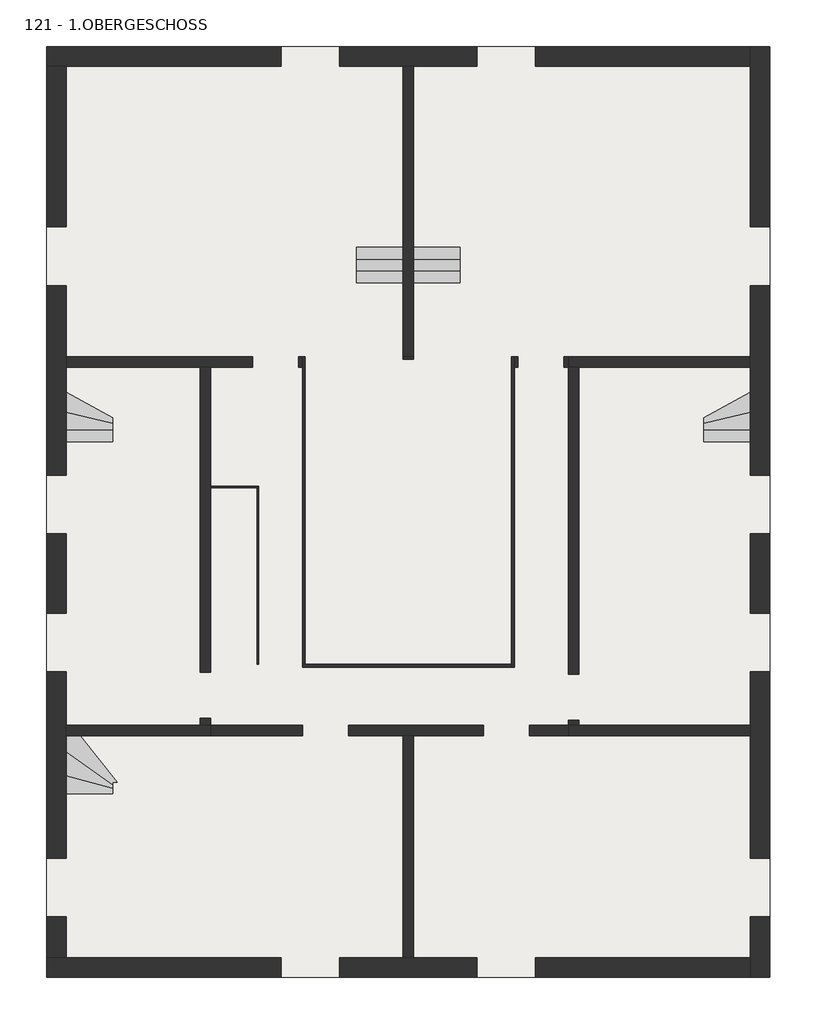
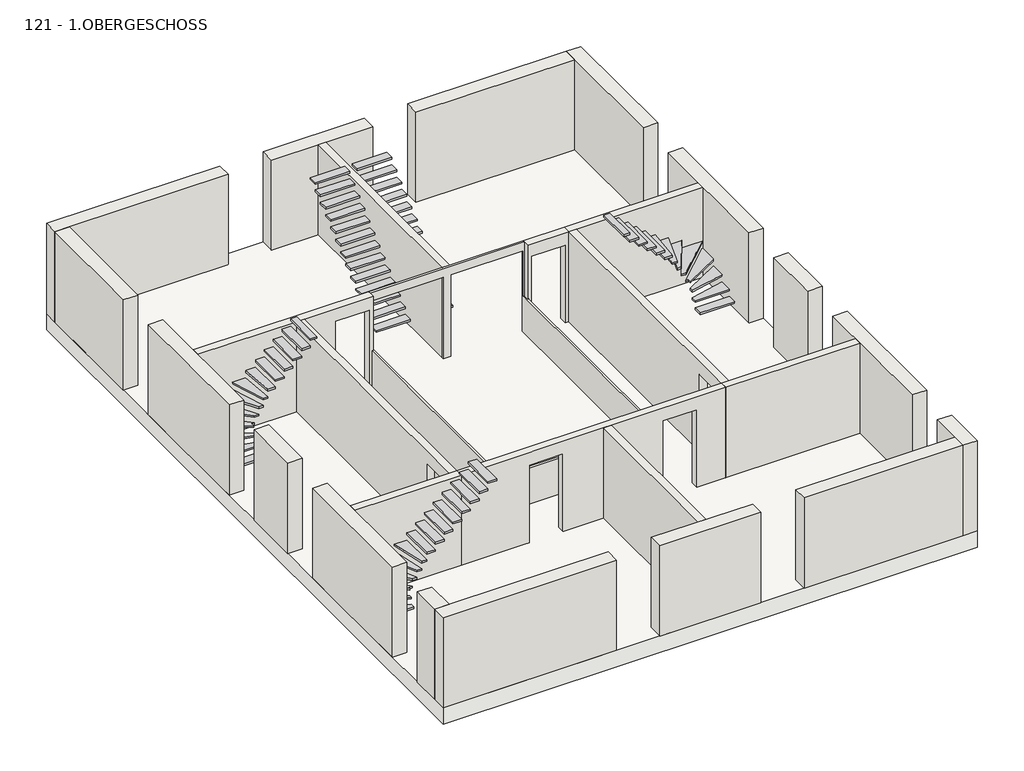
# One storey: 20 walls, 10 stairs, 1 slab.
# Revit data of these elements (continued)
# Type "  97010 :   97010" (continued)
#   HasNonSkidSurface = no
# Type "  97882 :   97882"
#   Abrechnungsart = "St"
#   Allright_Bauteil_ID = "0121Tre0785065280"
#   Codetext = "TR-MASSIV-GER\\"
#   Material = "Stahlbeton"
#   Objektname = "Treppe"
#   NameOverride = " "
#   Reference = "STB-Treppe"
#   ThermalTransmittance = 0.0000 BTU/(h·ft²·°F)
#   NosingLength = 0.000 m
#   NumberOfRiser = 14
#   NumberOfTreads = 13
#   RiserHeight = 2.021 m
#   TreadLength = 2.300 m
#   IsExternal = no
#   FireExit = no
#   HandicapAccessible = no
#   HasNonSkidSurface = no
# Type "  98300 :   98300"
#   Abrechnungsart = "St"
#   Allright_Bauteil_ID = "0121Tre0785065278"
#   Codetext = "TR-MASSIV-GER\\"
#   Material = "Stahlbeton"
#   Objektname = "Treppe"
#   NameOverride = " "
#   Reference = "STB-Treppe"
#   ThermalTransmittance = 0.0000 BTU/(h·ft²·°F)
#   NosingLength = 0.000 m
#   NumberOfRiser = 14
#   NumberOfTreads = 13
#   RiserHeight = 2.021 m
#   TreadLength = 2.300 m
#   IsExternal = no
#   FireExit = no
#   HandicapAccessible = no
#   HasNonSkidSurface = no
# Type "  98728 :   98728"
#   Abrechnungsart = "St"
#   Allright_Bauteil_ID = "0121Tre0785070507"
#   Material = "Stahlbeton"
#   Objektname = "Treppe"
#   NameOverride = " "
#   ThermalTransmittance = 0.0000 BTU/(h·ft²·°F)
#   NosingLength = 0.000 m
#   NumberOfRiser = 14
#   NumberOfTreads = 13
#   RiserHeight = 2.021 m
#   TreadLength = 2.300 m
#   IsExternal = no
#   FireExit = no
#   HandicapAccessible = no
#   HasNonSkidSurface = no
# Type "  99154 :   99154"
#   Abrechnungsart = "St"
#   Allright_Bauteil_ID = "0121Tre0785070829"
#   Material = "Stahlbeton"
#   Objektname = "Treppe"
#   NameOverride = " "
#   ThermalTransmittance = 0.0000 BTU/(h·ft²·°F)
#   NosingLength = 0.000 m
#   NumberOfRiser = 14
#   NumberOfTreads = 13
#   RiserHeight = 2.021 m
#   TreadLength = 2.300 m
#   IsExternal = no
#   FireExit = no
#   HandicapAccessible = no
#   HasNonSkidSurface = no
# Type "  149542 :   149542"
#   Abrechnungsart = "St"
#   Allright_Bauteil_ID = "0131Tre0659044515"
#   Material = "Stahlbeton"
#   Objektname = "Treppe"
#   NameOverride = " "
#   ThermalTransmittance = 0.0000 BTU/(h·ft²·°F)
#   NosingLength = 0.000 m
#   NumberOfRiser = 14
#   NumberOfTreads = 14
#   RiserHeight = 2.000 m
#   TreadLength = 2.300 m
#   IsExternal = no
#   FireExit = no
#   HandicapAccessible = no
#   HasNonSkidSurface = no
# Type "  150414 :   150414"
#   Abrechnungsart = "St"
#   Allright_Bauteil_ID = "0131Tre0659044575"
#   Codetext = "TR-MASSIV-GER\\"
#   Material = "Stahlbeton"
#   Objektname = "Treppe"
#   NameOverride = " "
#   Reference = "STB-Treppe"
#   ThermalTransmittance = 0.0000 BTU/(h·ft²·°F)
#   NosingLength = 0.000 m
#   NumberOfRiser = 14
#   NumberOfTreads = 13
#   RiserHeight = 2.021 m
#   TreadLength = 2.300 m
#   IsExternal = no
#   FireExit = no
#   HandicapAccessible = no
#   HasNonSkidSurface = no
# Type "  150832 :   150832"
#   Abrechnungsart = "St"
#   Allright_Bauteil_ID = "0131Tre0659044593"
#   Codetext = "TR-MASSIV-GER\\"
#   Material = "Stahlbeton"
#   Objektname = "Treppe"
#   NameOverride = " "
#   Reference = "STB-Treppe"
#   ThermalTransmittance = 0.0000 BTU/(h·ft²·°F)
#   NosingLength = 0.000 m
#   NumberOfRiser = 14
#   NumberOfTreads = 13
#   RiserHeight = 2.021 m
#   TreadLength = 2.300 m
#   IsExternal = no
#   FireExit = no
#   HandicapAccessible = no
#   HasNonSkidSurface = no
# Type "  151260 :   151260"
#   Abrechnungsart = "St"
#   Allright_Bauteil_ID = "0131Tre0659044533"
#   Material = "Stahlbeton"
#   Objektname = "Treppe"
#   NameOverride = " "
#   ThermalTransmittance = 0.0000 BTU/(h·ft²·°F)
#   NosingLength = 0.000 m
#   NumberOfRiser = 14
#   NumberOfTreads = 13
#   RiserHeight = 2.021 m
#   TreadLength = 2.300 m
#   IsExternal = no
#   FireExit = no
#   HandicapAccessible = no
#   HasNonSkidSurface = no
# Type "  151686 :   151686"
#   Abrechnungsart = "St"
#   Allright_Bauteil_ID = "0131Tre0659044570"
#   Material = "Stahlbeton"
#   Objektname = "Treppe"
#   NameOverride = " "
#   ThermalTransmittance = 0.0000 BTU/(h·ft²·°F)
#   NosingLength = 0.000 m
#   NumberOfRiser = 14
#   NumberOfTreads = 13
#   RiserHeight = 2.021 m
#   TreadLength = 2.300 m
#   IsExternal = no
#   FireExit = no
#   HandicapAccessible = no
#   HasNonSkidSurface = no
# Type " :1152"
#   Layers, outside or top first: 0.380 m "holzschalung" (function 1)
# Type " :1161"
#   Layers, outside or top first: 0.380 m "holzschalung" (function 1)
# Type " :1164"
#   Layers, outside or top first: 0.380 m "holzschalung" (function 1)
# Type " :1165"
#   Layers, outside or top first: 0.380 m "holzschalung" (function 1)
# Type " :1166"
#   Layers, outside or top first: 0.050 m "glas" (function 1)
# Type "Holzwand:1150"
#   ThermalTransmittance = 0.0000 BTU/(h·ft²·°F)
#   Combustible = no
#   Compartmentation = no
#   Layers, outside or top first: 0.200 m "holzschalung" (function 1)
# Type "Holzwand:1151"
#   ThermalTransmittance = 0.0000 BTU/(h·ft²·°F)
#   Combustible = no
#   Compartmentation = no
#   Layers, outside or top first: 0.200 m "holzschalung" (function 1)
# Type "Holzwand:1153"
#   ThermalTransmittance = 0.0000 BTU/(h·ft²·°F)
#   Combustible = no
#   Compartmentation = no
#   Layers, outside or top first: 0.200 m "holzschalung" (function 1)
# Type "Holzwand:1154"
#   ThermalTransmittance = 0.0000 BTU/(h·ft²·°F)
#   Combustible = no
#   Compartmentation = no
#   Layers, outside or top first: 0.030 m "holzschalung" (function 1)
# Type "Holzwand:1155"
#   ThermalTransmittance = 0.0000 BTU/(h·ft²·°F)
#   Combustible = no
#   Compartmentation = no
#   Layers, outside or top first: 0.030 m "holzschalung" (function 1)
# Type "Holzwand:1156"
#   ThermalTransmittance = 0.0000 BTU/(h·ft²·°F)
#   Combustible = no
#   Compartmentation = no
#   Layers, outside or top first: 0.200 m "holzschalung" (function 1)
# Type "Holzwand:1157"
#   ThermalTransmittance = 0.0000 BTU/(h·ft²·°F)
#   Combustible = no
#   Compartmentation = no
#   Layers, outside or top first: 0.200 m "holzschalung" (function 1)
# Type "Holzwand:1158"
#   ThermalTransmittance = 0.0000 BTU/(h·ft²·°F)
#   Combustible = no
#   Compartmentation = no
#   Layers, outside or top first: 0.200 m "holzschalung" (function 1)
# Type "Holzwand:1159"
#   ThermalTransmittance = 0.0000 BTU/(h·ft²·°F)
#   Combustible = no
#   Compartmentation = no
#   Layers, outside or top first: 0.200 m "holzschalung" (function 1)
# Type "Holzwand:1160"
#   ThermalTransmittance = 0.0000 BTU/(h·ft²·°F)
#   Combustible = no
#   Compartmentation = no
#   Layers, outside or top first: 0.200 m "holzschalung" (function 1)
# Type "Holzwand:1162"
#   ThermalTransmittance = 0.0000 BTU/(h·ft²·°F)
#   Combustible = no
#   Compartmentation = no
#   Layers, outside or top first: 0.200 m "holzschalung" (function 1)
# Type "Holzwand:1163"
#   ThermalTransmittance = 0.0000 BTU/(h·ft²·°F)
#   Combustible = no
#   Compartmentation = no
#   Layers, outside or top first: 0.200 m "holzschalung" (function 1)
# Type " :1167"
#   Layers, outside or top first: 0.050 m "holzschalung" (function 1)
# Type " :1168"
#   Layers, outside or top first: 0.050 m "holzschalung" (function 1)
# Type " :1169"
#   Layers, outside or top first: 0.050 m "holzschalung" (function 1)
# Element 1 (IfcSlab, "Holzdecke 176 : Holzdecke 176")
#   IFC Predefined Type = "FLOOR"
#   Export to IFC As = "ifcslab"
#   IfcGUID = "1_9Us2eVX4OuIZjhNyqdxW"
#   Phase Created = New Construction
#   Materials on its faces: "holzschalung"
# Element 2 (IfcStair, "  97010 :   97010")
#   IFC Predefined Type = "NOTDEFINED"
#   Export to IFC As = "ifcstair"
#   IfcGUID = "2ccaodaeb6QgHPV1d4NBnA"
#   Phase Created = New Construction
#   Materials on its faces: "weiss"
# Element 3 (IfcStair, "  97882 :   97882")
#   IFC Predefined Type = "STRAIGHT_RUN_STAIR"
#   Export to IFC As = "ifcstair"
#   IfcGUID = "1nghyUHoH9yBc_lxkBTUjw"
#   Phase Created = New Construction
#   Materials on its faces: "weiss"
# Element 4 (IfcStair, "  98300 :   98300")
#   IFC Predefined Type = "STRAIGHT_RUN_STAIR"
#   Export to IFC As = "ifcstair"
#   IfcGUID = "2AC_Gmfhz1LvYwUyPOxWan"
#   Phase Created = New Construction
#   Materials on its faces: "weiss"
# Element 5 (IfcStair, "  98728 :   98728")
#   IFC Predefined Type = "NOTDEFINED"
#   Export to IFC As = "ifcstair"
#   IfcGUID = "04Edcgbk9CPwWYiYhycXFf"
#   Phase Created = New Construction
#   Materials on its faces: "weiss"
# Element 6 (IfcStair, "  99154 :   99154")
#   IFC Predefined Type = "NOTDEFINED"
#   Export to IFC As = "ifcstair"
#   IfcGUID = "1azVXxNdn2POY9VYN93ccY"
#   Phase Created = New Construction
#   Materials on its faces: "weiss"
# Element 7 (IfcStair, "  149542 :   149542")
#   IFC Predefined Type = "NOTDEFINED"
#   Export to IFC As = "ifcstair"
#   IfcGUID = "1sH4rJKnLAFOtHPnXrLkif"
#   Phase Created = New Construction
#   Materials on its faces: "weiss"
# Element 8 (IfcStair, "  150414 :   150414")
#   IFC Predefined Type = "STRAIGHT_RUN_STAIR"
#   Export to IFC As = "ifcstair"
#   IfcGUID = "3fdccs_Mj1YAyFFpBc3gyk"
#   Phase Created = New Construction
#   Materials on its faces: "weiss"
# Element 9 (IfcStair, "  150832 :   150832")
#   IFC Predefined Type = "STRAIGHT_RUN_STAIR"
#   Export to IFC As = "ifcstair"
#   IfcGUID = "2szmEZdbD3KBDvfX1Sa6Vh"
#   Phase Created = New Construction
#   Materials on its faces: "weiss"
# Element 10 (IfcStair, "  151260 :   151260")
#   IFC Predefined Type = "NOTDEFINED"
#   Export to IFC As = "ifcstair"
#   IfcGUID = "1YKyaFTbr8YR41yGjubBsl"
#   Phase Created = New Construction
#   Materials on its faces: "weiss"
# Element 11 (IfcStair, "  151686 :   151686")
#   IFC Predefined Type = "NOTDEFINED"
#   Export to IFC As = "ifcstair"
#   IfcGUID = "2KPGRYHzzCygzBebAeLtPz"
#   Phase Created = New Construction
#   Materials on its faces: "weiss"
# Element 12 (IfcWall, " :1152")
#   Export to IFC As = "ifcwall"
#   IfcGUID = "2CeDj8YZTCPx$yj4WDVOez"
#   NameOverride = " "
#   Abrechnungsart = "m³"
#   Allright_Bauteil_ID = "0121HWa0785064286"
#   Layer #1:Object Layer Attributes #1:Abrechnungsart = "m²"
#   Layer #1:Object Layer Attributes #1:Allright_Bauteil_ID = "0121Wa 0785064367"
#   Layer #1:Object Layer Attributes #1:Gewerk = "Zimmer- und Holzbauarbeiten"
#   Layer #1:Object Layer Attributes #1:Material = "k.Ausw."
#   Layer #1:Object Layer Attributes #1:Objektname = "Wand"
#   Layer #1:Object Layer Attributes #1:Status = "Neubau"
#   MEP Wandtyp = "HO-WA-HSW\\"
#   Objektname = "Gesamtwand"
#   built-in parameter 1001111 = 0.505 m
#   Top Offset = 0.000 m
#   Base Offset = 0.505 m
#   Unconnected Height = 2.500 m
#   wall height = 2.500 m
#   Layer #1:Object Layer Attributes #1:2D Interaktion = yes
#   Phase Created = New Construction
#   Base Constraint = 121 - 1.OBERGESCHOSS
#   Materials on its faces: "holzschalung"
# Element 13 (IfcWall, " :1161")
#   Export to IFC As = "ifcwall"
#   IfcGUID = "2TnImcbz91shb3jN7Wgb8B"
#   Comments = "OG Sued"
#   Mark = "OG Sued"
#   NameOverride = " "
#   Abrechnungsart = "m³"
#   Allright_Bauteil_ID = "0121HWa0785064349"
#   Layer #1:Object Layer Attributes #1:Abrechnungsart = "m²"
#   Layer #1:Object Layer Attributes #1:Allright_Bauteil_ID = "0121Wa 0785064397"
#   Layer #1:Object Layer Attributes #1:Gewerk = "Zimmer- und Holzbauarbeiten"
#   Layer #1:Object Layer Attributes #1:Material = "k.Ausw."
#   Layer #1:Object Layer Attributes #1:Objektname = "Wand"
#   Layer #1:Object Layer Attributes #1:Status = "Neubau"
#   MEP Wandtyp = "HO-WA-HSW\\"
#   Objektname = "Gesamtwand"
#   built-in parameter 1001111 = 0.505 m
#   Top Offset = 0.000 m
#   Base Offset = 0.505 m
#   Unconnected Height = 2.500 m
#   wall height = 2.500 m
#   Layer #1:Object Layer Attributes #1:2D Interaktion = yes
#   Phase Created = New Construction
#   Base Constraint = 121 - 1.OBERGESCHOSS
#   Materials on its faces: "holzschalung"
# Element 14 (IfcWall, " :1164")
#   Export to IFC As = "ifcwall"
#   IfcGUID = "1tWRh4hxLAdASVw4VNE3to"
#   NameOverride = " "
#   Abrechnungsart = "m³"
#   Allright_Bauteil_ID = "0121HWa0785092952"
#   Layer #1:Object Layer Attributes #1:Abrechnungsart = "m²"
#   Layer #1:Object Layer Attributes #1:Allright_Bauteil_ID = "0121Wa 0785092986"
#   Layer #1:Object Layer Attributes #1:Gewerk = "Zimmer- und Holzbauarbeiten"
#   Layer #1:Object Layer Attributes #1:Material = "k.Ausw."
#   Layer #1:Object Layer Attributes #1:Objektname = "Wand"
#   Layer #1:Object Layer Attributes #1:Status = "Neubau"
#   MEP Wandtyp = "HO-WA-HSW\\"
#   Objektname = "Gesamtwand"
#   built-in parameter 1001111 = 0.505 m
#   Top Offset = 0.000 m
#   Base Offset = 0.505 m
#   Unconnected Height = 2.500 m
#   wall height = 2.500 m
#   Layer #1:Object Layer Attributes #1:2D Interaktion = yes
#   Phase Created = New Construction
#   Base Constraint = 121 - 1.OBERGESCHOSS
#   Materials on its faces: "holzschalung"
# Element 15 (IfcWall, " :1165")
#   Export to IFC As = "ifcwall"
#   IfcGUID = "1HE73MTmDEEBf4AV7ughZ8"
#   NameOverride = " "
#   Abrechnungsart = "m³"
#   Allright_Bauteil_ID = "0121HWa0785097898"
#   Layer #1:Object Layer Attributes #1:Abrechnungsart = "m²"
#   Layer #1:Object Layer Attributes #1:Allright_Bauteil_ID = "0121Wa 0785097934"
#   Layer #1:Object Layer Attributes #1:Gewerk = "Zimmer- und Holzbauarbeiten"
#   Layer #1:Object Layer Attributes #1:Material = "k.Ausw."
#   Layer #1:Object Layer Attributes #1:Objektname = "Wand"
#   Layer #1:Object Layer Attributes #1:Status = "Neubau"
#   MEP Wandtyp = "HO-WA-HSW\\"
#   Objektname = "Gesamtwand"
#   built-in parameter 1001111 = 0.505 m
#   Top Offset = 0.000 m
#   Base Offset = 0.505 m
#   Unconnected Height = 2.500 m
#   wall height = 2.500 m
#   Layer #1:Object Layer Attributes #1:2D Interaktion = yes
#   Phase Created = New Construction
#   Base Constraint = 121 - 1.OBERGESCHOSS
#   Materials on its faces: "holzschalung"
# Element 16 (IfcWall, " :1166")
#   Export to IFC As = "ifcwall"
#   IfcGUID = "0t2qqx1kvDZPNPdKl4bfzP"
#   NameOverride = " "
#   Abrechnungsart = "m³"
#   Allright_Bauteil_ID = "0121HWa0785064296"
#   Layer #1:Object Layer Attributes #1:Abrechnungsart = "m²"
#   Layer #1:Object Layer Attributes #1:Allright_Bauteil_ID = "0121Wa 0785064386"
#   Layer #1:Object Layer Attributes #1:Gewerk = "Zimmer- und Holzbauarbeiten"
#   Layer #1:Object Layer Attributes #1:Material = "k.Ausw."
#   Layer #1:Object Layer Attributes #1:Objektname = "Wand"
#   Layer #1:Object Layer Attributes #1:Status = "Neubau"
#   MEP Wandtyp = "HO-WA-HSW\\"
#   Objektname = "Gesamtwand"
#   built-in parameter 1001111 = 0.505 m
#   Top Offset = 0.000 m
#   Base Offset = 0.505 m
#   Unconnected Height = 2.500 m
#   wall height = 2.500 m
#   Layer #1:Object Layer Attributes #1:2D Interaktion = yes
#   Phase Created = New Construction
#   Base Constraint = 121 - 1.OBERGESCHOSS
#   Materials on its faces: "glas"
# Element 17 (IfcWall, "Holzwand:1150")
#   Export to IFC As = "ifcwall"
#   IfcGUID = "3nZ5Mon9nBjwoRgvyoor9a"
#   NameOverride = "Holzwand"
#   Abrechnungsart = "St"
#   Allright_Bauteil_ID = "0121HWa0785065367"
#   Bezeichnung = "Holzwand"
#   Layer #1:Object Layer Attributes #1:Abrechnungsart = "m²"
#   Layer #1:Object Layer Attributes #1:Allright_Bauteil_ID = "0121Wa 0785065369"
#   Layer #1:Object Layer Attributes #1:Bezeichnung = "Holzwand"
#   Layer #1:Object Layer Attributes #1:Codetext = "HO-WI-HSW\\"
#   Layer #1:Object Layer Attributes #1:Gewerk = "Zimmer- und Holzbauarbeiten"
#   Layer #1:Object Layer Attributes #1:Material = "Holz"
#   Layer #1:Object Layer Attributes #1:Objektname = "Wand"
#   Layer #1:Object Layer Attributes #1:Reference = "Holzwand"
#   Layer #1:Object Layer Attributes #1:Status = "Neubau"
#   MEP Wandtyp = "HO-WA-HSW\\"
#   Objektname = "Gesamtwand"
#   Reference = "Holzwand"
#   Status = "NEW"
#   built-in parameter 1001111 = 0.505 m
#   Top Offset = 0.000 m
#   Base Offset = 0.505 m
#   Unconnected Height = 2.500 m
#   wall height = 2.500 m
#   Layer #1:Object Layer Attributes #1:U-Wert = 0
#   Layer #1:Object Layer Attributes #1:2D Interaktion = yes
#   Layer #1:Object Layer Attributes #1:Außenbauteil = no
#   Layer #1:Object Layer Attributes #1:Brandabschnittsdefinierendes Bauteil = no
#   Layer #1:Object Layer Attributes #1:Brennbares Material = no
#   Layer #1:Object Layer Attributes #1:Raumhohe Wand = yes
#   Layer #1:Object Layer Attributes #1:Tragendes Bauteil = yes
#   ExtendToStructure = yes
#   IsExternal = no
#   LoadBearing = yes
#   Phase Created = New Construction
#   Base Constraint = 121 - 1.OBERGESCHOSS
#   Materials on its faces: "holzschalung"
# Element 18 (IfcWall, "Holzwand:1151")
#   Export to IFC As = "ifcwall"
#   IfcGUID = "3jE1E$NFj7vAP$vn70kdrt"
#   NameOverride = "Holzwand"
#   Abrechnungsart = "St"
#   Allright_Bauteil_ID = "0121HWa0785066899"
#   Bezeichnung = "Holzwand"
#   Layer #1:Object Layer Attributes #1:Abrechnungsart = "m²"
#   Layer #1:Object Layer Attributes #1:Allright_Bauteil_ID = "0121Wa 0785066901"
#   Layer #1:Object Layer Attributes #1:Bezeichnung = "Holzwand"
#   Layer #1:Object Layer Attributes #1:Codetext = "HO-WI-HSW\\"
#   Layer #1:Object Layer Attributes #1:Gewerk = "Zimmer- und Holzbauarbeiten"
#   Layer #1:Object Layer Attributes #1:Material = "Holz"
#   Layer #1:Object Layer Attributes #1:Objektname = "Wand"
#   Layer #1:Object Layer Attributes #1:Reference = "Holzwand"
#   Layer #1:Object Layer Attributes #1:Status = "Neubau"
#   MEP Wandtyp = "HO-WA-HSW\\"
#   Objektname = "Gesamtwand"
#   Reference = "Holzwand"
#   Status = "NEW"
#   built-in parameter 1001111 = 0.505 m
#   Top Offset = 0.000 m
#   Base Offset = 0.505 m
#   Unconnected Height = 2.500 m
#   wall height = 2.500 m
#   Layer #1:Object Layer Attributes #1:U-Wert = 0
#   Layer #1:Object Layer Attributes #1:2D Interaktion = yes
#   Layer #1:Object Layer Attributes #1:Außenbauteil = no
#   Layer #1:Object Layer Attributes #1:Brandabschnittsdefinierendes Bauteil = no
#   Layer #1:Object Layer Attributes #1:Brennbares Material = no
#   Layer #1:Object Layer Attributes #1:Raumhohe Wand = yes
#   Layer #1:Object Layer Attributes #1:Tragendes Bauteil = yes
#   ExtendToStructure = yes
#   IsExternal = no
#   LoadBearing = yes
#   Phase Created = New Construction
#   Base Constraint = 121 - 1.OBERGESCHOSS
#   Materials on its faces: "holzschalung"
# Element 19 (IfcWall, "Holzwand:1153")
#   Export to IFC As = "ifcwall"
#   IfcGUID = "1Zhxv5EALB9e6_$pCtUEXg"
#   NameOverride = "Holzwand"
#   Abrechnungsart = "St"
#   Allright_Bauteil_ID = "0121HWa0785065540"
#   Bezeichnung = "Holzwand"
#   Layer #1:Object Layer Attributes #1:Abrechnungsart = "m²"
#   Layer #1:Object Layer Attributes #1:Allright_Bauteil_ID = "0121Wa 0785065541"
#   Layer #1:Object Layer Attributes #1:Bezeichnung = "Holzwand"
#   Layer #1:Object Layer Attributes #1:Codetext = "HO-WI-HSW\\"
#   Layer #1:Object Layer Attributes #1:Gewerk = "Zimmer- und Holzbauarbeiten"
#   Layer #1:Object Layer Attributes #1:Material = "Holz"
#   Layer #1:Object Layer Attributes #1:Objektname = "Wand"
#   Layer #1:Object Layer Attributes #1:Reference = "Holzwand"
#   Layer #1:Object Layer Attributes #1:Status = "Neubau"
#   MEP Wandtyp = "HO-WA-HSW\\"
#   Objektname = "Gesamtwand"
#   Reference = "Holzwand"
#   Status = "NEW"
#   built-in parameter 1001111 = 0.505 m
#   Top Offset = 0.000 m
#   Base Offset = 0.505 m
#   Unconnected Height = 2.500 m
#   wall height = 2.500 m
#   Layer #1:Object Layer Attributes #1:U-Wert = 0
#   Layer #1:Object Layer Attributes #1:2D Interaktion = yes
#   Layer #1:Object Layer Attributes #1:Außenbauteil = no
#   Layer #1:Object Layer Attributes #1:Brandabschnittsdefinierendes Bauteil = no
#   Layer #1:Object Layer Attributes #1:Brennbares Material = no
#   Layer #1:Object Layer Attributes #1:Raumhohe Wand = yes
#   Layer #1:Object Layer Attributes #1:Tragendes Bauteil = yes
#   ExtendToStructure = yes
#   IsExternal = no
#   LoadBearing = yes
#   Phase Created = New Construction
#   Base Constraint = 121 - 1.OBERGESCHOSS
#   Materials on its faces: "holzschalung"
# Element 20 (IfcWall, "Holzwand:1154")
#   Export to IFC As = "ifcwall"
#   IfcGUID = "2MsVq3EJn0K8wHdQ6uoxnd"
#   NameOverride = "Holzwand"
#   Abrechnungsart = "St"
#   Allright_Bauteil_ID = "0121HWa0785067355"
#   Bezeichnung = "Holzwand"
#   Layer #1:Object Layer Attributes #1:Abrechnungsart = "m²"
#   Layer #1:Object Layer Attributes #1:Allright_Bauteil_ID = "0121Wa 0785067356"
#   Layer #1:Object Layer Attributes #1:Codetext = "HO-WI-HSW\\"
#   Layer #1:Object Layer Attributes #1:Gewerk = "Zimmer- und Holzbauarbeiten"
#   Layer #1:Object Layer Attributes #1:Material = "Holz"
#   Layer #1:Object Layer Attributes #1:Objektname = "Wand"
#   Layer #1:Object Layer Attributes #1:Reference = "Holzwand"
#   Layer #1:Object Layer Attributes #1:Status = "Neubau"
#   MEP Wandtyp = "HO-WA-HSW\\"
#   Objektname = "Gesamtwand"
#   Reference = "Holzwand"
#   Status = "NEW"
#   built-in parameter 1001111 = 0.505 m
#   Top Offset = 0.000 m
#   Base Offset = 0.505 m
#   Unconnected Height = 1.000 m
#   wall height = 1.000 m
#   Layer #1:Object Layer Attributes #1:U-Wert = 0
#   Layer #1:Object Layer Attributes #1:2D Interaktion = yes
#   Layer #1:Object Layer Attributes #1:Außenbauteil = no
#   Layer #1:Object Layer Attributes #1:Brandabschnittsdefinierendes Bauteil = no
#   Layer #1:Object Layer Attributes #1:Brennbares Material = no
#   Layer #1:Object Layer Attributes #1:Raumhohe Wand = yes
#   ExtendToStructure = yes
#   IsExternal = no
#   LoadBearing = yes
#   Phase Created = New Construction
#   Base Constraint = 121 - 1.OBERGESCHOSS
#   Materials on its faces: "holzschalung"
# Element 21 (IfcWall, "Holzwand:1155")
#   Export to IFC As = "ifcwall"
#   IfcGUID = "1F_ySrDsP9oP3MqXymSTVO"
#   NameOverride = "Holzwand"
#   Abrechnungsart = "St"
#   Allright_Bauteil_ID = "0121HWa0785067347"
#   Bezeichnung = "Holzwand"
#   Layer #1:Object Layer Attributes #1:Abrechnungsart = "m²"
#   Layer #1:Object Layer Attributes #1:Allright_Bauteil_ID = "0121Wa 0785067348"
#   Layer #1:Object Layer Attributes #1:Codetext = "HO-WI-HSW\\"
#   Layer #1:Object Layer Attributes #1:Gewerk = "Zimmer- und Holzbauarbeiten"
#   Layer #1:Object Layer Attributes #1:Material = "Holz"
#   Layer #1:Object Layer Attributes #1:Objektname = "Wand"
#   Layer #1:Object Layer Attributes #1:Reference = "Holzwand"
#   Layer #1:Object Layer Attributes #1:Status = "Neubau"
#   MEP Wandtyp = "HO-WA-HSW\\"
#   Objektname = "Gesamtwand"
#   Reference = "Holzwand"
#   Status = "NEW"
#   built-in parameter 1001111 = 0.505 m
#   Top Offset = 0.000 m
#   Base Offset = 0.505 m
#   Unconnected Height = 1.000 m
#   wall height = 1.000 m
#   Layer #1:Object Layer Attributes #1:U-Wert = 0
#   Layer #1:Object Layer Attributes #1:2D Interaktion = yes
#   Layer #1:Object Layer Attributes #1:Außenbauteil = no
#   Layer #1:Object Layer Attributes #1:Brandabschnittsdefinierendes Bauteil = no
#   Layer #1:Object Layer Attributes #1:Brennbares Material = no
#   Layer #1:Object Layer Attributes #1:Raumhohe Wand = yes
#   ExtendToStructure = yes
#   IsExternal = no
#   LoadBearing = yes
#   Phase Created = New Construction
#   Base Constraint = 121 - 1.OBERGESCHOSS
#   Materials on its faces: "holzschalung"
# Element 22 (IfcWall, "Holzwand:1156")
#   Export to IFC As = "ifcwall"
#   IfcGUID = "0gtwZwppj1pObqyI7HY41_"
#   NameOverride = "Holzwand"
#   Abrechnungsart = "St"
#   Allright_Bauteil_ID = "0121HWa0785064323"
#   Bezeichnung = "Holzwand"
#   Layer #1:Object Layer Attributes #1:Abrechnungsart = "m²"
#   Layer #1:Object Layer Attributes #1:Allright_Bauteil_ID = "0121Wa 0785064369"
#   Layer #1:Object Layer Attributes #1:Bezeichnung = "Holzwand"
#   Layer #1:Object Layer Attributes #1:Codetext = "HO-WI-HSW\\"
#   Layer #1:Object Layer Attributes #1:Gewerk = "Zimmer- und Holzbauarbeiten"
#   Layer #1:Object Layer Attributes #1:Material = "Holz"
#   Layer #1:Object Layer Attributes #1:Objektname = "Wand"
#   Layer #1:Object Layer Attributes #1:Reference = "Holzwand"
#   Layer #1:Object Layer Attributes #1:Status = "Neubau"
#   MEP Wandtyp = "HO-WA-HSW\\"
#   Objektname = "Gesamtwand"
#   Reference = "Holzwand"
#   Status = "NEW"
#   built-in parameter 1001111 = 0.505 m
#   Top Offset = 0.000 m
#   Base Offset = 0.505 m
#   Unconnected Height = 2.500 m
#   wall height = 2.500 m
#   Layer #1:Object Layer Attributes #1:U-Wert = 0
#   Layer #1:Object Layer Attributes #1:2D Interaktion = yes
#   Layer #1:Object Layer Attributes #1:Außenbauteil = no
#   Layer #1:Object Layer Attributes #1:Brandabschnittsdefinierendes Bauteil = no
#   Layer #1:Object Layer Attributes #1:Brennbares Material = no
#   Layer #1:Object Layer Attributes #1:Raumhohe Wand = yes
#   Layer #1:Object Layer Attributes #1:Tragendes Bauteil = yes
#   ExtendToStructure = yes
#   IsExternal = no
#   LoadBearing = yes
#   Phase Created = New Construction
#   Base Constraint = 121 - 1.OBERGESCHOSS
#   Materials on its faces: "holzschalung"
# Element 23 (IfcWall, "Holzwand:1157")
#   Export to IFC As = "ifcwall"
#   IfcGUID = "0tY6$O1l121AktLhYSWZjf"
#   NameOverride = "Holzwand"
#   Abrechnungsart = "St"
#   Allright_Bauteil_ID = "0121HWa0785064381"
#   Bezeichnung = "Holzwand"
#   Layer #1:Object Layer Attributes #1:Abrechnungsart = "m²"
#   Layer #1:Object Layer Attributes #1:Allright_Bauteil_ID = "0121Wa 0785064384"
#   Layer #1:Object Layer Attributes #1:Bezeichnung = "Holzwand"
#   Layer #1:Object Layer Attributes #1:Codetext = "HO-WI-HSW\\"
#   Layer #1:Object Layer Attributes #1:Gewerk = "Zimmer- und Holzbauarbeiten"
#   Layer #1:Object Layer Attributes #1:Material = "Holz"
#   Layer #1:Object Layer Attributes #1:Objektname = "Wand"
#   Layer #1:Object Layer Attributes #1:Reference = "Holzwand"
#   Layer #1:Object Layer Attributes #1:Status = "Neubau"
#   MEP Wandtyp = "HO-WA-HSW\\"
#   Objektname = "Gesamtwand"
#   Reference = "Holzwand"
#   Status = "NEW"
#   built-in parameter 1001111 = 0.505 m
#   Top Offset = 0.000 m
#   Base Offset = 0.505 m
#   Unconnected Height = 2.500 m
#   wall height = 2.500 m
#   Layer #1:Object Layer Attributes #1:U-Wert = 0
#   Layer #1:Object Layer Attributes #1:2D Interaktion = yes
#   Layer #1:Object Layer Attributes #1:Außenbauteil = no
#   Layer #1:Object Layer Attributes #1:Brandabschnittsdefinierendes Bauteil = no
#   Layer #1:Object Layer Attributes #1:Brennbares Material = no
#   Layer #1:Object Layer Attributes #1:Raumhohe Wand = yes
#   Layer #1:Object Layer Attributes #1:Tragendes Bauteil = yes
#   ExtendToStructure = yes
#   IsExternal = no
#   LoadBearing = yes
#   Phase Created = New Construction
#   Base Constraint = 121 - 1.OBERGESCHOSS
#   Materials on its faces: "holzschalung"
# Element 24 (IfcWall, "Holzwand:1158")
#   Export to IFC As = "ifcwall"
#   IfcGUID = "2Mr8L52dj4iP8MoJTiOa9p"
#   NameOverride = "Holzwand"
#   Abrechnungsart = "St"
#   Allright_Bauteil_ID = "0121HWa0785069286"
#   Bezeichnung = "Holzwand"
#   Layer #1:Object Layer Attributes #1:Abrechnungsart = "m²"
#   Layer #1:Object Layer Attributes #1:Allright_Bauteil_ID = "0121Wa 0785069294"
#   Layer #1:Object Layer Attributes #1:Bezeichnung = "Holzwand"
#   Layer #1:Object Layer Attributes #1:Codetext = "HO-WI-HSW\\"
#   Layer #1:Object Layer Attributes #1:Gewerk = "Zimmer- und Holzbauarbeiten"
#   Layer #1:Object Layer Attributes #1:Material = "Holz"
#   Layer #1:Object Layer Attributes #1:Objektname = "Wand"
#   Layer #1:Object Layer Attributes #1:Reference = "Holzwand"
#   Layer #1:Object Layer Attributes #1:Status = "Neubau"
#   MEP Wandtyp = "HO-WA-HSW\\"
#   Objektname = "Gesamtwand"
#   Reference = "Holzwand"
#   Status = "NEW"
#   built-in parameter 1001111 = 0.505 m
#   Top Offset = 0.000 m
#   Base Offset = 0.505 m
#   Unconnected Height = 2.500 m
#   wall height = 2.500 m
#   Layer #1:Object Layer Attributes #1:U-Wert = 0
#   Layer #1:Object Layer Attributes #1:2D Interaktion = yes
#   Layer #1:Object Layer Attributes #1:Außenbauteil = no
#   Layer #1:Object Layer Attributes #1:Brandabschnittsdefinierendes Bauteil = no
#   Layer #1:Object Layer Attributes #1:Brennbares Material = no
#   Layer #1:Object Layer Attributes #1:Raumhohe Wand = yes
#   Layer #1:Object Layer Attributes #1:Tragendes Bauteil = yes
#   ExtendToStructure = yes
#   IsExternal = no
#   LoadBearing = yes
#   Phase Created = New Construction
#   Base Constraint = 121 - 1.OBERGESCHOSS
#   Materials on its faces: "holzschalung"
# Element 25 (IfcWall, "Holzwand:1159")
#   Export to IFC As = "ifcwall"
#   IfcGUID = "36leNf4gL9OB_v358ffY76"
#   NameOverride = "Holzwand"
#   Abrechnungsart = "St"
#   Allright_Bauteil_ID = "0121HWa0785064324"
#   Bezeichnung = "Holzwand"
#   Layer #1:Object Layer Attributes #1:Abrechnungsart = "m²"
#   Layer #1:Object Layer Attributes #1:Allright_Bauteil_ID = "0121Wa 0785064395"
#   Layer #1:Object Layer Attributes #1:Bezeichnung = "Holzwand"
#   Layer #1:Object Layer Attributes #1:Codetext = "HO-WI-HSW\\"
#   Layer #1:Object Layer Attributes #1:Gewerk = "Zimmer- und Holzbauarbeiten"
#   Layer #1:Object Layer Attributes #1:Material = "Holz"
#   Layer #1:Object Layer Attributes #1:Objektname = "Wand"
#   Layer #1:Object Layer Attributes #1:Reference = "Holzwand"
#   Layer #1:Object Layer Attributes #1:Status = "Neubau"
#   MEP Wandtyp = "HO-WA-HSW\\"
#   Objektname = "Gesamtwand"
#   Reference = "Holzwand"
#   Status = "NEW"
#   built-in parameter 1001111 = 0.505 m
#   Top Offset = 0.000 m
#   Base Offset = 0.505 m
#   Unconnected Height = 2.500 m
#   wall height = 2.500 m
#   Layer #1:Object Layer Attributes #1:U-Wert = 0
#   Layer #1:Object Layer Attributes #1:2D Interaktion = yes
#   Layer #1:Object Layer Attributes #1:Außenbauteil = no
#   Layer #1:Object Layer Attributes #1:Brandabschnittsdefinierendes Bauteil = no
#   Layer #1:Object Layer Attributes #1:Brennbares Material = no
#   Layer #1:Object Layer Attributes #1:Raumhohe Wand = yes
#   Layer #1:Object Layer Attributes #1:Tragendes Bauteil = yes
#   ExtendToStructure = yes
#   IsExternal = no
#   LoadBearing = yes
#   Phase Created = New Construction
#   Base Constraint = 121 - 1.OBERGESCHOSS
#   Materials on its faces: "holzschalung"
# Element 26 (IfcWall, "Holzwand:1160")
#   Export to IFC As = "ifcwall"
#   IfcGUID = "3kHHpx_NTE_9JnfL3dFkYB"
#   NameOverride = "Holzwand"
#   Abrechnungsart = "St"
#   Allright_Bauteil_ID = "0121HWa0785064389"
#   Bezeichnung = "Holzwand"
#   Layer #1:Object Layer Attributes #1:Abrechnungsart = "m²"
#   Layer #1:Object Layer Attributes #1:Allright_Bauteil_ID = "0121Wa 0785064393"
#   Layer #1:Object Layer Attributes #1:Bezeichnung = "Holzwand"
#   Layer #1:Object Layer Attributes #1:Codetext = "HO-WI-HSW\\"
#   Layer #1:Object Layer Attributes #1:Gewerk = "Zimmer- und Holzbauarbeiten"
#   Layer #1:Object Layer Attributes #1:Material = "Holz"
#   Layer #1:Object Layer Attributes #1:Objektname = "Wand"
#   Layer #1:Object Layer Attributes #1:Reference = "Holzwand"
#   Layer #1:Object Layer Attributes #1:Status = "Neubau"
#   MEP Wandtyp = "HO-WA-HSW\\"
#   Objektname = "Gesamtwand"
#   Reference = "Holzwand"
#   Status = "NEW"
#   built-in parameter 1001111 = 0.505 m
#   Top Offset = 0.000 m
#   Base Offset = 0.505 m
#   Unconnected Height = 2.500 m
#   wall height = 2.500 m
#   Layer #1:Object Layer Attributes #1:U-Wert = 0
#   Layer #1:Object Layer Attributes #1:2D Interaktion = yes
#   Layer #1:Object Layer Attributes #1:Außenbauteil = no
#   Layer #1:Object Layer Attributes #1:Brandabschnittsdefinierendes Bauteil = no
#   Layer #1:Object Layer Attributes #1:Brennbares Material = no
#   Layer #1:Object Layer Attributes #1:Raumhohe Wand = yes
#   Layer #1:Object Layer Attributes #1:Tragendes Bauteil = yes
#   ExtendToStructure = yes
#   IsExternal = no
#   LoadBearing = yes
#   Phase Created = New Construction
#   Base Constraint = 121 - 1.OBERGESCHOSS
#   Materials on its faces: "holzschalung"
# Element 27 (IfcWall, "Holzwand:1162")
#   Export to IFC As = "ifcwall"
#   IfcGUID = "26lQuimMP00PZvPhbBRI2R"
#   NameOverride = "Holzwand"
#   Abrechnungsart = "St"
#   Allright_Bauteil_ID = "0121HWa0785065329"
#   Bezeichnung = "Holzwand"
#   Layer #1:Object Layer Attributes #1:Abrechnungsart = "m²"
#   Layer #1:Object Layer Attributes #1:Allright_Bauteil_ID = "0121Wa 0785065331"
#   Layer #1:Object Layer Attributes #1:Bezeichnung = "Holzwand"
#   Layer #1:Object Layer Attributes #1:Codetext = "HO-WI-HSW\\"
#   Layer #1:Object Layer Attributes #1:Gewerk = "Zimmer- und Holzbauarbeiten"
#   Layer #1:Object Layer Attributes #1:Material = "Holz"
#   Layer #1:Object Layer Attributes #1:Objektname = "Wand"
#   Layer #1:Object Layer Attributes #1:Reference = "Holzwand"
#   Layer #1:Object Layer Attributes #1:Status = "Neubau"
#   MEP Wandtyp = "HO-WA-HSW\\"
#   Objektname = "Gesamtwand"
#   Reference = "Holzwand"
#   Status = "NEW"
#   built-in parameter 1001111 = 0.505 m
#   Top Offset = 0.000 m
#   Base Offset = 0.505 m
#   Unconnected Height = 2.500 m
#   wall height = 2.500 m
#   Layer #1:Object Layer Attributes #1:U-Wert = 0
#   Layer #1:Object Layer Attributes #1:2D Interaktion = yes
#   Layer #1:Object Layer Attributes #1:Außenbauteil = no
#   Layer #1:Object Layer Attributes #1:Brandabschnittsdefinierendes Bauteil = no
#   Layer #1:Object Layer Attributes #1:Brennbares Material = no
#   Layer #1:Object Layer Attributes #1:Raumhohe Wand = yes
#   Layer #1:Object Layer Attributes #1:Tragendes Bauteil = yes
#   ExtendToStructure = yes
#   IsExternal = no
#   LoadBearing = yes
#   Phase Created = New Construction
#   Base Constraint = 121 - 1.OBERGESCHOSS
#   Materials on its faces: "holzschalung"
# Element 28 (IfcWall, "Holzwand:1163")
#   Export to IFC As = "ifcwall"
#   IfcGUID = "3atU$IMTH8YP$GZozT8ehc"
#   NameOverride = "Holzwand"
#   Abrechnungsart = "St"
#   Allright_Bauteil_ID = "0121HWa0785064334"
#   Bezeichnung = "Holzwand"
#   Layer #1:Object Layer Attributes #1:Abrechnungsart = "m²"
#   Layer #1:Object Layer Attributes #1:Allright_Bauteil_ID = "0121Wa 0785064371"
#   Layer #1:Object Layer Attributes #1:Bezeichnung = "Holzwand"
#   Layer #1:Object Layer Attributes #1:Codetext = "HO-WI-HSW\\"
#   Layer #1:Object Layer Attributes #1:Gewerk = "Zimmer- und Holzbauarbeiten"
#   Layer #1:Object Layer Attributes #1:Material = "Holz"
#   Layer #1:Object Layer Attributes #1:Objektname = "Wand"
#   Layer #1:Object Layer Attributes #1:Reference = "Holzwand"
#   Layer #1:Object Layer Attributes #1:Status = "Neubau"
#   MEP Wandtyp = "HO-WA-HSW\\"
#   Objektname = "Gesamtwand"
#   Reference = "Holzwand"
#   Status = "NEW"
#   built-in parameter 1001111 = 0.505 m
#   Top Offset = 0.000 m
#   Base Offset = 0.505 m
#   Unconnected Height = 2.500 m
#   wall height = 2.500 m
#   Layer #1:Object Layer Attributes #1:U-Wert = 0
#   Layer #1:Object Layer Attributes #1:2D Interaktion = yes
#   Layer #1:Object Layer Attributes #1:Außenbauteil = no
#   Layer #1:Object Layer Attributes #1:Brandabschnittsdefinierendes Bauteil = no
#   Layer #1:Object Layer Attributes #1:Brennbares Material = no
#   Layer #1:Object Layer Attributes #1:Raumhohe Wand = yes
#   Layer #1:Object Layer Attributes #1:Tragendes Bauteil = yes
#   ExtendToStructure = yes
#   IsExternal = no
#   LoadBearing = yes
#   Phase Created = New Construction
#   Base Constraint = 121 - 1.OBERGESCHOSS
#   Materials on its faces: "holzschalung"
# Element 29 (IfcWall, " :1167")
#   Export to IFC As = "ifcwall"
#   IfcGUID = "35Iolt9MTFw82QPYPk5JvU"
#   NameOverride = " "
#   Abrechnungsart = "m³"
#   Allright_Bauteil_ID = "0121HWa0785064294"
#   Layer #1:Object Layer Attributes #1:Abrechnungsart = "m²"
#   Layer #1:Object Layer Attributes #1:Allright_Bauteil_ID = "0121Wa 0785064340"
#   Layer #1:Object Layer Attributes #1:Gewerk = "Zimmer- und Holzbauarbeiten"
#   Layer #1:Object Layer Attributes #1:Material = "k.Ausw."
#   Layer #1:Object Layer Attributes #1:Objektname = "Wand"
#   Layer #1:Object Layer Attributes #1:Status = "Neubau"
#   MEP Wandtyp = "HO-WA-HSW\\"
#   Objektname = "Gesamtwand"
#   built-in parameter 1001111 = 0.505 m
#   Top Offset = 0.000 m
#   Base Offset = 0.505 m
#   Unconnected Height = 1.000 m
#   wall height = 1.000 m
#   Layer #1:Object Layer Attributes #1:2D Interaktion = yes
#   Layer #1:Object Layer Attributes #1:Tragendes Bauteil = no
#   Phase Created = New Construction
#   Base Constraint = 121 - 1.OBERGESCHOSS
#   Materials on its faces: "holzschalung", "glas"
# Element 30 (IfcWall, " :1168")
#   Export to IFC As = "ifcwall"
#   IfcGUID = "21NDiotIv7sAO2c5Bbio25"
#   NameOverride = " "
#   Abrechnungsart = "m³"
#   Allright_Bauteil_ID = "0121HWa0785064290"
#   Layer #1:Object Layer Attributes #1:Abrechnungsart = "m²"
#   Layer #1:Object Layer Attributes #1:Allright_Bauteil_ID = "0121Wa 0785064348"
#   Layer #1:Object Layer Attributes #1:Gewerk = "Zimmer- und Holzbauarbeiten"
#   Layer #1:Object Layer Attributes #1:Material = "k.Ausw."
#   Layer #1:Object Layer Attributes #1:Objektname = "Wand"
#   Layer #1:Object Layer Attributes #1:Status = "Neubau"
#   MEP Wandtyp = "HO-WA-HSW\\"
#   Objektname = "Gesamtwand"
#   built-in parameter 1001111 = 0.505 m
#   Top Offset = 0.000 m
#   Base Offset = 0.505 m
#   Unconnected Height = 1.000 m
#   wall height = 1.000 m
#   Layer #1:Object Layer Attributes #1:2D Interaktion = yes
#   Layer #1:Object Layer Attributes #1:Tragendes Bauteil = no
#   Phase Created = New Construction
#   Base Constraint = 121 - 1.OBERGESCHOSS
#   Materials on its faces: "holzschalung"
# Element 31 (IfcWall, " :1169")
#   Export to IFC As = "ifcwall"
#   IfcGUID = "2aL_F8tebFMgUeEEKPH5KO"
#   NameOverride = " "
#   Abrechnungsart = "m³"
#   Allright_Bauteil_ID = "0121HWa0785064292"
#   Layer #1:Object Layer Attributes #1:Abrechnungsart = "m²"
#   Layer #1:Object Layer Attributes #1:Allright_Bauteil_ID = "0121Wa 0785064346"
#   Layer #1:Object Layer Attributes #1:Gewerk = "Zimmer- und Holzbauarbeiten"
#   Layer #1:Object Layer Attributes #1:Material = "k.Ausw."
#   Layer #1:Object Layer Attributes #1:Objektname = "Wand"
#   Layer #1:Object Layer Attributes #1:Status = "Neubau"
#   MEP Wandtyp = "HO-WA-HSW\\"
#   Objektname = "Gesamtwand"
#   built-in parameter 1001111 = 0.505 m
#   Top Offset = 0.000 m
#   Base Offset = 0.505 m
#   Unconnected Height = 1.000 m
#   wall height = 1.000 m
#   Layer #1:Object Layer Attributes #1:2D Interaktion = yes
#   Layer #1:Object Layer Attributes #1:Tragendes Bauteil = no
#   Phase Created = New Construction
#   Base Constraint = 121 - 1.OBERGESCHOSS
#   Materials on its faces: "holzschalung", "glas"
# Materials
#   "holzschalung": class "Unassigned", colour RGB 128 128 128, transparency 0
#   "glas": class "Unassigned", colour RGB 250 253 254, transparency 0.95
#   "weiss": class "Unassigned", colour RGB 255 255 255, transparency 0
# Room at (13460, 8317.808) mm, phase "New Construction", upper offset 2.500 m, lower offset 0.000 m
#   Export to IFC As = "ifcspace"
#   IfcGUID = "3ldkF51q96e9r6BFrUoGvb"
#   Comments = ""
#   Number = "30"
#   Name = "Zimmer 4"
#   Abrechnungsart = "m²"
#   Allright_Bauteil_ID = "0121Rau0785070860"
#   Objektname = "Raum"
#   Status = "Neubau"
#   Flächenart_DIN277 = "N"
#   Flächenart_Wohnfläche = "WO"
#   Nutzungsart_Din277 = "NUF"
#   Ortscode_Geschoßbezeichnung = "OG"
#   Raumumschließung = "R"
#   Faktor_DIN277 = 1
#   Faktor_Wohnfläche_Raum = 1
#   BauNVO_Anrechnung_auf_GF = 0
#   BauNVO_Anrechnung_auf_GR = 0
#   Raum unter Treppe (Wohnfl erst ab 2m) = 0
# Room at (3177.5, 8317.808) mm, phase "New Construction", upper offset 2.500 m, lower offset 0.000 m
#   Export to IFC As = "ifcspace"
#   IfcGUID = "0$kYsoxCXA3h__RP_0NR6Q"
#   Comments = ""
#   Number = "31"
#   Name = "Zimmer 7"
#   Abrechnungsart = "m²"
#   Allright_Bauteil_ID = "0121Rau0785070777"
#   Objektname = "Raum"
#   Status = "Neubau"
#   Flächenart_DIN277 = "N"
#   Flächenart_Wohnfläche = "WO"
#   Nutzungsart_Din277 = "NUF"
#   Ortscode_Geschoßbezeichnung = "OG"
#   Raumumschließung = "R"
#   Faktor_DIN277 = 1
#   Faktor_Wohnfläche_Raum = 1
#   BauNVO_Anrechnung_auf_GF = 0
#   BauNVO_Anrechnung_auf_GR = 0
#   Raum unter Treppe (Wohnfl erst ab 2m) = 0
# Room, not placed, phase "New Construction", upper offset 0.000 m, lower offset 0.000 m
#   Export to IFC As = "ifcspace"
#   IfcGUID = "2dgNyc8bb9E9nVZAdiTRxB"
#   Comments = ""
#   Number = "32"
#   Name = "Zimmer 2"
#   Abrechnungsart = "m²"
#   Allright_Bauteil_ID = "0121Rau0785090661"
#   Objektname = "Raum"
#   Status = "Neubau"
#   Flächenart_DIN277 = "N"
#   Flächenart_Wohnfläche = "WO"
#   Nutzungsart_Din277 = "NUF"
#   Ortscode_Geschoßbezeichnung = "OG"
#   Raumumschließung = "R"
#   Faktor_DIN277 = 1
#   Faktor_Wohnfläche_Raum = 1
#   BauNVO_Anrechnung_auf_GF = 0
#   BauNVO_Anrechnung_auf_GR = 0
#   Raum unter Treppe (Wohnfl erst ab 2m) = 0
# Room, not placed, phase "New Construction", upper offset 0.000 m, lower offset 0.000 m
#   Export to IFC As = "ifcspace"
#   IfcGUID = "1tzfmU$RP7LfmN2qGRU1XT"
#   Comments = ""
#   Number = "33"
#   Name = "Zimmer 3"
#   Abrechnungsart = "m²"
#   Allright_Bauteil_ID = "0121Rau0785090678"
#   Objektname = "Raum"
#   Status = "Neubau"
#   Flächenart_DIN277 = "N"
#   Flächenart_Wohnfläche = "WO"
#   Nutzungsart_Din277 = "NUF"
#   Ortscode_Geschoßbezeichnung = "OG"
#   Raumumschließung = "R"
#   Faktor_DIN277 = 1
#   Faktor_Wohnfläche_Raum = 1
#   BauNVO_Anrechnung_auf_GF = 0
#   BauNVO_Anrechnung_auf_GR = 0
#   Raum unter Treppe (Wohnfl erst ab 2m) = 0
# Room at (10648.317, 16360) mm, phase "New Construction", upper offset 2.500 m, lower offset 0.000 m
#   Export to IFC As = "ifcspace"
#   IfcGUID = "27JspUp7H1Z9DG3JvgTQFt"
#   Comments = ""
#   Number = "34"
#   Name = "Zimmer 5"
#   Abrechnungsart = "m²"
#   Allright_Bauteil_ID = "0121Rau0785066391"
#   Objektname = "Raum"
#   Status = "Neubau"
#   Flächenart_DIN277 = "N"
#   Flächenart_Wohnfläche = "WO"
#   Nutzungsart_Din277 = "NUF"
#   Ortscode_Geschoßbezeichnung = "OG"
#   Raumumschließung = "R"
#   Faktor_DIN277 = 1
#   Faktor_Wohnfläche_Raum = 1
#   BauNVO_Anrechnung_auf_GF = 0
#   BauNVO_Anrechnung_auf_GR = 0
#   Raum unter Treppe (Wohnfl erst ab 2m) = 0
# Room, not placed, phase "New Construction", upper offset 0.000 m, lower offset 0.000 m
#   Export to IFC As = "ifcspace"
#   IfcGUID = "2t08KtCRDEo9EvknasL6lQ"
#   Comments = ""
#   Number = "35"
#   Name = "Flur OG"
#   Abrechnungsart = "m²"
#   Allright_Bauteil_ID = "0121Rau0785066415"
#   Objektname = "Raum"
#   Status = "Neubau"
#   Flächenart_DIN277 = "N"
#   Flächenart_Wohnfläche = "WO"
#   Nutzungsart_Din277 = "NUF"
#   Ortscode_Geschoßbezeichnung = "OG"
#   Raumumschließung = "R"
#   Faktor_DIN277 = 1
#   Faktor_Wohnfläche_Raum = 1
#   BauNVO_Anrechnung_auf_GF = 0
#   BauNVO_Anrechnung_auf_GR = 0
#   Raum unter Treppe (Wohnfl erst ab 2m) = 0
# Room at (3928.317, 16360) mm, phase "New Construction", upper offset 2.500 m, lower offset 0.000 m
#   Export to IFC As = "ifcspace"
#   IfcGUID = "3J0l6V$An1WgW4ojn5k9EU"
#   Comments = ""
#   Number = "36"
#   Name = "Zimmer 6"
#   Abrechnungsart = "m²"
#   Allright_Bauteil_ID = "0121Rau0785066399"
#   Objektname = "Raum"
#   Status = "Neubau"
#   Flächenart_DIN277 = "N"
#   Flächenart_Wohnfläche = "WO"
#   Nutzungsart_Din277 = "NUF"
#   Ortscode_Geschoßbezeichnung = "OG"
#   Raumumschließung = "R"
#   Faktor_DIN277 = 1
#   Faktor_Wohnfläche_Raum = 1
#   BauNVO_Anrechnung_auf_GF = 0
#   BauNVO_Anrechnung_auf_GR = 0
#   Raum unter Treppe (Wohnfl erst ab 2m) = 0
